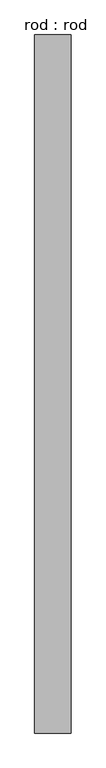
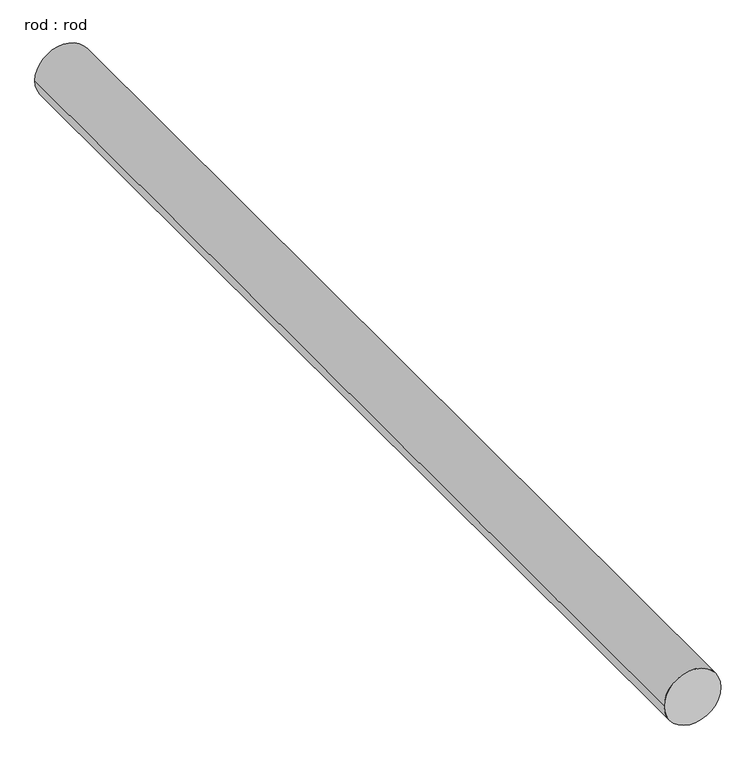
"""IFC4 building model written with IfcOpenShell, lengths in millimetres: proxy geometry, rod : rod."""

from ifc_helpers import new_model, si_unit, point, frame, frame_2d, origin, place, context, project, spatial, circle_curve, trimmed, segment, composite_curve, outline, extrude, source, transform, mapped, element, save


def rod_rod_8ce2bf8d(model_context):
    return source(origin(), model_context, "Body", "SweptSolid", [
        extrude(outline(composite_curve([segment(trimmed(circle_curve(frame_2d((0.0108462, 0.0)), 200.0), [point((0.0108462, 200.0))], [point((0.0108462, -200.0))], False, "CARTESIAN"), True, "CONTINUOUS"), segment(trimmed(circle_curve(frame_2d((0.0108462, 0.0)), 200.0), [point((0.0108462, -200.0))], [point((0.0108462, 200.0))], False, "CARTESIAN"), True, "CONTINUOUS")], self_intersect=False)), frame((0.0, 261.20492, 0.0), z_axis=(0.0, 1.0, 0.0), x_axis=(0.0, 0.0, 1.0)), (0.0, 0.0, 1.0), 7663.0473907),
    ])


if __name__ == "__main__":
    model = new_model("IFC4")
    model_context = context("Model", 3, world=origin())
    ifc_project = project(units=[si_unit("LENGTHUNIT", "METRE", prefix="MILLI")], contexts=[model_context])
    site = spatial("IfcSite", under=ifc_project)
    building = spatial("IfcBuilding", under=site)
    placement = place(None, origin())
    rod_rod_shape = rod_rod_8ce2bf8d(model_context)
    element("IfcBuildingElementProxy", 1, Name="rod : rod", ObjectType="rod : rod", at=placement, inside=building, context=model_context, shape_type="MappedRepresentation", body=[
        mapped(rod_rod_shape, transform((0.0, 0.0, 0.0), x_axis=(1.0, 0.0, 0.0), y_axis=(0.0, 1.0, 0.0), z_axis=(0.0, 0.0, 1.0))),
    ])
    save(model, "model.ifc")

# Revit data of these elements
# Type "rod : rod"
#   Default Elevation = 0
